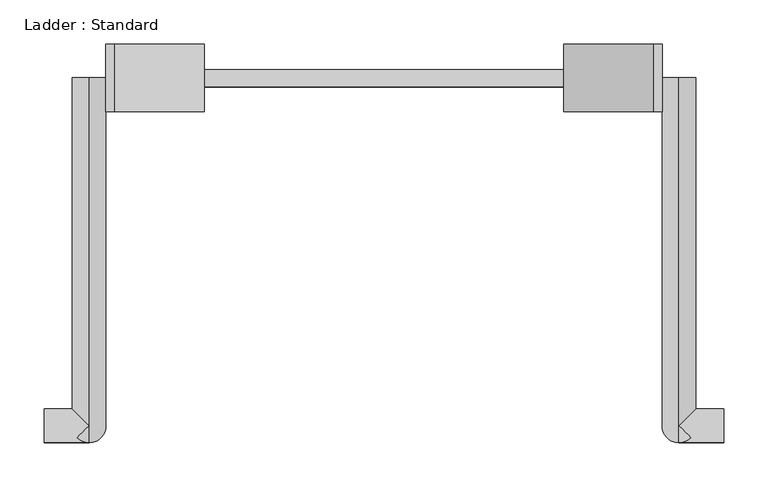
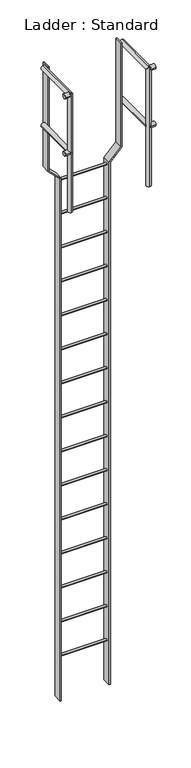
"""IFC4 building model written with IfcOpenShell, lengths in millimetres: proxy geometry, Ladder : Standard."""

import ifcopenshell
import ifcopenshell.guid

model = None  # the IFC model being written
_history = None  # IfcOwnerHistory: only IFC2X3 demands one
_inside = {}  # id of a spatial element -> (the spatial element, [elements in it])
_under = {}  # id of a project, library or spatial element -> (it, [spatial elements below it])
_declared = {}  # id of a project -> (the project, [libraries it declares])
_typed = {}  # id of a type object -> (the type object, [elements of that type])
_made_of = {}  # id of a material, layer set ... -> (it, [elements and type objects made of it])


def new_model(schema):
    """Start an empty IFC model of exactly this schema.

    Asked for "IFC4X3", IfcOpenShell would pick the latest addendum, in which some entities
    have other attributes; the version numbers below select the first issue.
    IFC2X3 requires an IfcOwnerHistory on every rooted entity: one is made here for all.
    """
    global model, _history
    if schema == "IFC4X3":
        model = ifcopenshell.file(schema_version=(4, 3, 0, 0))
    else:
        model = ifcopenshell.file(schema=schema)
    _inside.clear()
    _under.clear()
    _declared.clear()
    _typed.clear()
    _made_of.clear()
    _history = None
    if model.schema == "IFC2X3":
        org = make("IfcOrganization", Name="unknown")
        user = make(
            "IfcPersonAndOrganization",
            ThePerson=make("IfcPerson", FamilyName="unknown"),
            TheOrganization=org,
        )
        app = make(
            "IfcApplication",
            ApplicationDeveloper=org,
            Version="unknown",
            ApplicationFullName="unknown",
            ApplicationIdentifier="unknown",
        )
        _history = make(
            "IfcOwnerHistory",
            OwningUser=user,
            OwningApplication=app,
            ChangeAction="ADDED",
            CreationDate=0,
        )
    return model


def make(cls, **values):
    """One entity of the class cls with the attributes given. An attribute that is None is left unset."""
    return model.create_entity(
        cls, **{name: value for name, value in values.items() if value is not None}
    )


def rooted(cls, **values):
    """An entity with a GlobalId (a new one), such as an element, a storey or a relation."""
    return make(cls, GlobalId=ifcopenshell.guid.new(), OwnerHistory=_history, **values)


def si_unit(unit_type, name, prefix=None):
    """IfcSIUnit, for example si_unit("LENGTHUNIT", "METRE", prefix="MILLI")."""
    return make("IfcSIUnit", UnitType=unit_type, Prefix=prefix, Name=name)


def assignment(units):
    """IfcUnitAssignment: the units of a project."""
    return None if units is None else make("IfcUnitAssignment", Units=units)


def point(xyz):
    """IfcCartesianPoint."""
    return None if xyz is None else make("IfcCartesianPoint", Coordinates=xyz)


def direction(xyz):
    """IfcDirection."""
    return None if xyz is None else make("IfcDirection", DirectionRatios=xyz)


def frame(location, z_axis=None, x_axis=None):
    """IfcAxis2Placement3D, a coordinate frame: its origin and axes. An axis left out is left unset."""
    return make(
        "IfcAxis2Placement3D",
        Location=point(location),
        Axis=direction(z_axis),
        RefDirection=direction(x_axis),
    )


def frame_2d(location, x_axis=None):
    """IfcAxis2Placement2D, a coordinate frame in the plane: its origin and x axis."""
    return make(
        "IfcAxis2Placement2D", Location=point(location), RefDirection=direction(x_axis)
    )


def origin():
    """The frame at (0, 0, 0) with its axes left unset."""
    return frame((0.0, 0.0, 0.0))


def place(relative_to, where):
    """IfcLocalPlacement: puts the frame where relative to a parent placement (None: the world)."""
    return make(
        "IfcLocalPlacement", PlacementRelTo=relative_to, RelativePlacement=where
    )


def context(
    kind, dimensions, precision=None, world=None, true_north=None, identifier=None
):
    """IfcGeometricRepresentationContext, for example the 3D "Model" context."""
    return make(
        "IfcGeometricRepresentationContext",
        ContextIdentifier=identifier,
        ContextType=kind,
        CoordinateSpaceDimension=dimensions,
        Precision=precision,
        WorldCoordinateSystem=world,
        TrueNorth=true_north,
    )


def project(units=None, contexts=None):
    """IfcProject with its units and contexts."""
    return rooted(
        "IfcProject",
        Name="project",
        RepresentationContexts=contexts,
        UnitsInContext=assignment(units),
    )


def spatial(cls, under=None, at=None, **own):
    """A site, building, storey or space (cls), placed at a placement, below another one or the project."""
    s = rooted(cls, ObjectPlacement=at, **own)
    if under is not None:
        _under.setdefault(under.id(), (under, []))[1].append(s)
    return s


def polyline(points):
    """IfcPolyline through the points."""
    return make("IfcPolyline", Points=[point(p) for p in points])


def circle_curve(where, radius):
    """IfcCircle in the frame where."""
    return make("IfcCircle", Position=where, Radius=radius)


def ellipse_curve(where, semi_axis1, semi_axis2):
    """IfcEllipse in the frame where."""
    return make(
        "IfcEllipse", Position=where, SemiAxis1=semi_axis1, SemiAxis2=semi_axis2
    )


def trimmed(basis, trim1, trim2, sense, master):
    """IfcTrimmedCurve: the piece of a basis curve between two trims."""
    return make(
        "IfcTrimmedCurve",
        BasisCurve=basis,
        Trim1=trim1,
        Trim2=trim2,
        SenseAgreement=sense,
        MasterRepresentation=master,
    )


def segment(curve, same_sense, transition):
    """IfcCompositeCurveSegment."""
    return make(
        "IfcCompositeCurveSegment",
        Transition=transition,
        SameSense=same_sense,
        ParentCurve=curve,
    )


def composite_curve(segments, self_intersect=None):
    """IfcCompositeCurve: segments joined end to end."""
    return make("IfcCompositeCurve", Segments=segments, SelfIntersect=self_intersect)


def outline(outer, holes=None, kind="AREA"):
    """IfcArbitraryClosedProfileDef: a profile drawn as a closed curve; with holes, ...WithVoids."""
    if holes is None:
        return make("IfcArbitraryClosedProfileDef", ProfileType=kind, OuterCurve=outer)
    return make(
        "IfcArbitraryProfileDefWithVoids",
        ProfileType=kind,
        OuterCurve=outer,
        InnerCurves=holes,
    )


def extrude(swept, where, along, depth):
    """IfcExtrudedAreaSolid: the profile swept, set in the frame where, extruded along a direction by depth."""
    return make(
        "IfcExtrudedAreaSolid",
        SweptArea=swept,
        Position=where,
        ExtrudedDirection=direction(along),
        Depth=depth,
    )


def shape(context_of_items, identifier, shape_type, items):
    """IfcShapeRepresentation: the items that make up one representation, for example the "Body"."""
    return make(
        "IfcShapeRepresentation",
        ContextOfItems=context_of_items,
        RepresentationIdentifier=identifier,
        RepresentationType=shape_type,
        Items=items,
    )


def source(mapping_origin, context_of_items, identifier, shape_type, items):
    """IfcRepresentationMap: a shape defined once, which mapped items show again and again."""
    return make(
        "IfcRepresentationMap",
        MappingOrigin=mapping_origin,
        MappedRepresentation=shape(context_of_items, identifier, shape_type, items),
    )


def transform(
    local_origin,
    x_axis=None,
    y_axis=None,
    z_axis=None,
    scale=None,
    scale2=None,
    scale3=None,
    uniform=True,
):
    """IfcCartesianTransformationOperator3D, or its non-uniform kind. x_axis, y_axis, z_axis: its Axis1, 2, 3."""
    if uniform:
        return make(
            "IfcCartesianTransformationOperator3D",
            Axis1=direction(x_axis),
            Axis2=direction(y_axis),
            LocalOrigin=point(local_origin),
            Scale=scale,
            Axis3=direction(z_axis),
        )
    return make(
        "IfcCartesianTransformationOperator3DnonUniform",
        Axis1=direction(x_axis),
        Axis2=direction(y_axis),
        LocalOrigin=point(local_origin),
        Scale=scale,
        Axis3=direction(z_axis),
        Scale2=scale2,
        Scale3=scale3,
    )


def mapped(mapping_source, mapping_target):
    """IfcMappedItem: shows the shape of a source again, moved by a transform."""
    return make(
        "IfcMappedItem", MappingSource=mapping_source, MappingTarget=mapping_target
    )


def made_of(thing, what):
    """Note that an element or type object is made of a material, layer set ...; save() writes the relation."""
    if what is not None:
        _made_of.setdefault(what.id(), (what, []))[1].append(thing)
    return thing


def element(
    cls,
    number,
    at=None,
    inside=None,
    cuts=None,
    type_object=None,
    material=None,
    context=None,
    identifier="Body",
    shape_type=None,
    held_by="IfcProductDefinitionShape",
    body=None,
    shapes=None,
    **own,
):
    """One element of the class cls, such as IfcWall. Its Tag is "e" and its number.

    at: its placement. inside: the storey or other place that contains it. cuts: it is an
    opening in that element (IfcRelVoidsElement). A single representation is given by context,
    identifier, shape_type and body (its items); several are given by shapes. held_by: the class
    of the entity that holds the representations. save() writes the other relations.
    """
    e = rooted(cls, Tag="e%d" % number, ObjectPlacement=at, **own)
    if body is not None:
        shapes = [shape(context, identifier, shape_type, body)]
    if shapes is not None:
        e.Representation = make(held_by, Representations=shapes)
    if inside is not None:
        _inside.setdefault(inside.id(), (inside, []))[1].append(e)
    if cuts is not None:
        rooted(
            "IfcRelVoidsElement", RelatingBuildingElement=cuts, RelatedOpeningElement=e
        )
    if type_object is not None:
        _typed.setdefault(type_object.id(), (type_object, []))[1].append(e)
    return made_of(e, material)


def aggregate(whole, parts):
    """IfcRelAggregates: a whole, such as a stair, and the parts it consists of."""
    return rooted("IfcRelAggregates", RelatingObject=whole, RelatedObjects=parts)


def save(model, path):
    """Write the relations noted so far, then the file.

    IfcRelAggregates (storeys below a building ...), IfcRelContainedInSpatialStructure (elements
    in a storey), IfcRelDefinesByType, IfcRelAssociatesMaterial and IfcRelDeclares: one each for
    every whole, place, type object, material and project.
    """
    for whole, parts in _under.values():
        aggregate(whole, parts)
    for where, things in _inside.values():
        rooted(
            "IfcRelContainedInSpatialStructure",
            RelatedElements=things,
            RelatingStructure=where,
        )
    for kind, things in _typed.values():
        rooted("IfcRelDefinesByType", RelatedObjects=things, RelatingType=kind)
    for what, things in _made_of.values():
        rooted("IfcRelAssociatesMaterial", RelatedObjects=things, RelatingMaterial=what)
    for by, libraries in _declared.values():
        rooted("IfcRelDeclares", RelatingContext=by, RelatedDefinitions=libraries)
    model.write(path)


def plane_surface(at):
    """IfcPlane: the flat surface through the origin of the frame at, square to its z axis."""
    return make("IfcPlane", Position=at)


def cylinder_surface(at, radius):
    """IfcCylindricalSurface: all points at the distance radius from the z axis of the frame at."""
    return make("IfcCylindricalSurface", Position=at, Radius=radius)


def advanced_brep(points, edges, surfaces, faces):
    """IfcAdvancedBrep: a solid bounded by faces that lie on surfaces and meet in shared edges.

    An edge is (start, end): straight between two places in points (the first is 0);
    or (start, end, curve); or (start, end, curve, False) where it runs against its curve.
    A face is (place in surfaces, loops), or (place, loops, False) where it looks against
    its surface's normal. A loop lists edges by number (the first is 1), with a minus sign
    where the edge is run from its end to its start. The first loop is the outer one.
    """
    corners = [point(p) for p in points]
    vertices = [make("IfcVertexPoint", VertexGeometry=c) for c in corners]
    made = []
    for start, end, *more in edges:
        made.append(
            make(
                "IfcEdgeCurve",
                EdgeStart=vertices[start],
                EdgeEnd=vertices[end],
                EdgeGeometry=more[0] if more else make("IfcPolyline", Points=[corners[start], corners[end]]),
                SameSense=more[1] if len(more) > 1 else True,
            )
        )
    hull = []
    for where, loops, *sense in faces:
        bounds = []
        for j, loop in enumerate(loops):
            ring = [make("IfcOrientedEdge", EdgeElement=made[abs(k) - 1], Orientation=k > 0) for k in loop]
            bounds.append(
                make(
                    "IfcFaceOuterBound" if j == 0 else "IfcFaceBound",
                    Bound=make("IfcEdgeLoop", EdgeList=ring),
                    Orientation=True,
                )
            )
        hull.append(make("IfcAdvancedFace", Bounds=bounds, FaceSurface=surfaces[where], SameSense=sense[0] if sense else True))
    return make("IfcAdvancedBrep", Outer=make("IfcClosedShell", CfsFaces=hull))


def ladder_standard_9d180ee5(model_context):
    return source(origin(), model_context, "Body", "SolidModel", [
        extrude(outline(composite_curve([segment(trimmed(circle_curve(frame_2d((393.7, -4267.2)), 9.525), [point((384.175, -4267.2))], [point((403.225, -4267.2))], False, "CARTESIAN"), True, "CONTINUOUS"), segment(trimmed(circle_curve(frame_2d((393.7, -4267.2)), 9.525), [point((403.225, -4267.2))], [point((384.175, -4267.2))], False, "CARTESIAN"), True, "CONTINUOUS")], self_intersect=False)), frame((-203.2, 0.0, 0.0), z_axis=(1.0, 0.0, 0.0), x_axis=(0.0, 1.0, 0.0)), (0.0, 0.0, 1.0), 406.4),
        extrude(outline(composite_curve([segment(trimmed(circle_curve(frame_2d((393.7, -3962.4)), 9.525), [point((384.175, -3962.4))], [point((403.225, -3962.4))], False, "CARTESIAN"), True, "CONTINUOUS"), segment(trimmed(circle_curve(frame_2d((393.7, -3962.4)), 9.525), [point((403.225, -3962.4))], [point((384.175, -3962.4))], False, "CARTESIAN"), True, "CONTINUOUS")], self_intersect=False)), frame((-203.2, 0.0, 0.0), z_axis=(1.0, 0.0, 0.0), x_axis=(0.0, 1.0, 0.0)), (0.0, 0.0, 1.0), 406.4),
        extrude(outline(composite_curve([segment(trimmed(circle_curve(frame_2d((393.7, -3657.6)), 9.525), [point((384.175, -3657.6))], [point((403.225, -3657.6))], False, "CARTESIAN"), True, "CONTINUOUS"), segment(trimmed(circle_curve(frame_2d((393.7, -3657.6)), 9.525), [point((403.225, -3657.6))], [point((384.175, -3657.6))], False, "CARTESIAN"), True, "CONTINUOUS")], self_intersect=False)), frame((-203.2, 0.0, 0.0), z_axis=(1.0, 0.0, 0.0), x_axis=(0.0, 1.0, 0.0)), (0.0, 0.0, 1.0), 406.4),
        extrude(outline(composite_curve([segment(trimmed(circle_curve(frame_2d((393.7, -3352.8)), 9.525), [point((384.175, -3352.8))], [point((403.225, -3352.8))], False, "CARTESIAN"), True, "CONTINUOUS"), segment(trimmed(circle_curve(frame_2d((393.7, -3352.8)), 9.525), [point((403.225, -3352.8))], [point((384.175, -3352.8))], False, "CARTESIAN"), True, "CONTINUOUS")], self_intersect=False)), frame((-203.2, 0.0, 0.0), z_axis=(1.0, 0.0, 0.0), x_axis=(0.0, 1.0, 0.0)), (0.0, 0.0, 1.0), 406.4),
        extrude(outline(composite_curve([segment(trimmed(circle_curve(frame_2d((393.7, -3048.0)), 9.525), [point((384.175, -3048.0))], [point((403.225, -3048.0))], False, "CARTESIAN"), True, "CONTINUOUS"), segment(trimmed(circle_curve(frame_2d((393.7, -3048.0)), 9.525), [point((403.225, -3048.0))], [point((384.175, -3048.0))], False, "CARTESIAN"), True, "CONTINUOUS")], self_intersect=False)), frame((-203.2, 0.0, 0.0), z_axis=(1.0, 0.0, 0.0), x_axis=(0.0, 1.0, 0.0)), (0.0, 0.0, 1.0), 406.4),
        extrude(outline(composite_curve([segment(trimmed(circle_curve(frame_2d((393.7, -2743.2)), 9.525), [point((384.175, -2743.2))], [point((403.225, -2743.2))], False, "CARTESIAN"), True, "CONTINUOUS"), segment(trimmed(circle_curve(frame_2d((393.7, -2743.2)), 9.525), [point((403.225, -2743.2))], [point((384.175, -2743.2))], False, "CARTESIAN"), True, "CONTINUOUS")], self_intersect=False)), frame((-203.2, 0.0, 0.0), z_axis=(1.0, 0.0, 0.0), x_axis=(0.0, 1.0, 0.0)), (0.0, 0.0, 1.0), 406.4),
        extrude(outline(composite_curve([segment(trimmed(circle_curve(frame_2d((393.7, -2438.4)), 9.525), [point((384.175, -2438.4))], [point((403.225, -2438.4))], False, "CARTESIAN"), True, "CONTINUOUS"), segment(trimmed(circle_curve(frame_2d((393.7, -2438.4)), 9.525), [point((403.225, -2438.4))], [point((384.175, -2438.4))], False, "CARTESIAN"), True, "CONTINUOUS")], self_intersect=False)), frame((-203.2, 0.0, 0.0), z_axis=(1.0, 0.0, 0.0), x_axis=(0.0, 1.0, 0.0)), (0.0, 0.0, 1.0), 406.4),
        extrude(outline(composite_curve([segment(trimmed(circle_curve(frame_2d((393.7, -2133.6)), 9.525), [point((384.175, -2133.6))], [point((403.225, -2133.6))], False, "CARTESIAN"), True, "CONTINUOUS"), segment(trimmed(circle_curve(frame_2d((393.7, -2133.6)), 9.525), [point((403.225, -2133.6))], [point((384.175, -2133.6))], False, "CARTESIAN"), True, "CONTINUOUS")], self_intersect=False)), frame((-203.2, 0.0, 0.0), z_axis=(1.0, 0.0, 0.0), x_axis=(0.0, 1.0, 0.0)), (0.0, 0.0, 1.0), 406.4),
        extrude(outline(composite_curve([segment(trimmed(circle_curve(frame_2d((393.7, -1828.8)), 9.525), [point((384.175, -1828.8))], [point((403.225, -1828.8))], False, "CARTESIAN"), True, "CONTINUOUS"), segment(trimmed(circle_curve(frame_2d((393.7, -1828.8)), 9.525), [point((403.225, -1828.8))], [point((384.175, -1828.8))], False, "CARTESIAN"), True, "CONTINUOUS")], self_intersect=False)), frame((-203.2, 0.0, 0.0), z_axis=(1.0, 0.0, 0.0), x_axis=(0.0, 1.0, 0.0)), (0.0, 0.0, 1.0), 406.4),
        extrude(outline(composite_curve([segment(trimmed(circle_curve(frame_2d((393.7, -1524.0)), 9.525), [point((384.175, -1524.0))], [point((403.225, -1524.0))], False, "CARTESIAN"), True, "CONTINUOUS"), segment(trimmed(circle_curve(frame_2d((393.7, -1524.0)), 9.525), [point((403.225, -1524.0))], [point((384.175, -1524.0))], False, "CARTESIAN"), True, "CONTINUOUS")], self_intersect=False)), frame((-203.2, 0.0, 0.0), z_axis=(1.0, 0.0, 0.0), x_axis=(0.0, 1.0, 0.0)), (0.0, 0.0, 1.0), 406.4),
        extrude(outline(composite_curve([segment(trimmed(circle_curve(frame_2d((393.7, -1219.2)), 9.525), [point((384.175, -1219.2))], [point((403.225, -1219.2))], False, "CARTESIAN"), True, "CONTINUOUS"), segment(trimmed(circle_curve(frame_2d((393.7, -1219.2)), 9.525), [point((403.225, -1219.2))], [point((384.175, -1219.2))], False, "CARTESIAN"), True, "CONTINUOUS")], self_intersect=False)), frame((-203.2, 0.0, 0.0), z_axis=(1.0, 0.0, 0.0), x_axis=(0.0, 1.0, 0.0)), (0.0, 0.0, 1.0), 406.4),
        extrude(outline(composite_curve([segment(trimmed(circle_curve(frame_2d((393.7, -914.4)), 9.525), [point((384.175, -914.4))], [point((403.225, -914.4))], False, "CARTESIAN"), True, "CONTINUOUS"), segment(trimmed(circle_curve(frame_2d((393.7, -914.4)), 9.525), [point((403.225, -914.4))], [point((384.175, -914.4))], False, "CARTESIAN"), True, "CONTINUOUS")], self_intersect=False)), frame((-203.2, 0.0, 0.0), z_axis=(1.0, 0.0, 0.0), x_axis=(0.0, 1.0, 0.0)), (0.0, 0.0, 1.0), 406.4),
        extrude(outline(composite_curve([segment(trimmed(circle_curve(frame_2d((393.7, -609.6)), 9.525), [point((384.175, -609.6))], [point((403.225, -609.6))], False, "CARTESIAN"), True, "CONTINUOUS"), segment(trimmed(circle_curve(frame_2d((393.7, -609.6)), 9.525), [point((403.225, -609.6))], [point((384.175, -609.6))], False, "CARTESIAN"), True, "CONTINUOUS")], self_intersect=False)), frame((-203.2, 0.0, 0.0), z_axis=(1.0, 0.0, 0.0), x_axis=(0.0, 1.0, 0.0)), (0.0, 0.0, 1.0), 406.4),
        extrude(outline(composite_curve([segment(trimmed(circle_curve(frame_2d((393.7, -304.8)), 9.525), [point((384.175, -304.8))], [point((403.225, -304.8))], False, "CARTESIAN"), True, "CONTINUOUS"), segment(trimmed(circle_curve(frame_2d((393.7, -304.8)), 9.525), [point((403.225, -304.8))], [point((384.175, -304.8))], False, "CARTESIAN"), True, "CONTINUOUS")], self_intersect=False)), frame((-203.2, 0.0, 0.0), z_axis=(1.0, 0.0, 0.0), x_axis=(0.0, 1.0, 0.0)), (0.0, 0.0, 1.0), 406.4),
        extrude(outline(composite_curve([segment(trimmed(circle_curve(frame_2d((393.7, 0.0)), 9.525), [point((384.175, 0.0))], [point((403.225, 0.0))], False, "CARTESIAN"), True, "CONTINUOUS"), segment(trimmed(circle_curve(frame_2d((393.7, 0.0)), 9.525), [point((403.225, 0.0))], [point((384.175, 0.0))], False, "CARTESIAN"), True, "CONTINUOUS")], self_intersect=False)), frame((-203.2, 0.0, 0.0), z_axis=(1.0, 0.0, 0.0), x_axis=(0.0, 1.0, 0.0)), (0.0, 0.0, 1.0), 406.4),
        advanced_brep(
        [(314.325, 393.7, 533.4), (352.425, 393.7, 533.4), (352.425, 19.05, 533.4), (346.8453842, 13.4703842, 519.9296158), (333.375, 19.05, 514.35), (314.325, 0.0, 533.4), (333.375, 19.05, 552.45), (346.8453842, 13.4703842, 546.8703842), (384.175, -19.05, 533.4), (384.175, 19.05, 533.4), (333.375, -19.05, 533.4), (333.375, 19.05, 0.0), (333.375, -19.05, 0.0), (333.375, 19.05, 1028.7), (346.8453842, 13.4703842, 1034.2796158), (333.375, -19.05, 1047.75), (346.8453842, -13.4703842, 1061.2203842), (333.375, -19.05, 1066.8), (333.375, 393.7, 1028.7), (333.375, 393.7, 1066.8), (333.375, 0.0, 1066.8), (352.425, 19.05, 1047.75), (384.175, -19.05, 1047.75), (384.175, 19.05, 1047.75)],
        [
            (0, 1, circle_curve(frame((333.375, 393.7, 533.4), z_axis=(0.0, 1.0, 0.0), x_axis=(1.0, 0.0, 0.0)), 19.05)),
            (1, 0, circle_curve(frame((333.375, 393.7, 533.4), z_axis=(0.0, 1.0, 0.0), x_axis=(1.0, 0.0, 0.0)), 19.05)),
            (1, 2),
            (2, 3, ellipse_curve(frame((333.375, 0.0, 533.4), z_axis=(-0.7071067811865459, 0.7071067811865492, 0.0), x_axis=(-0.7071067811865492, -0.7071067811865457, 0.0)), 26.9407684, 19.05)),
            (3, 4, ellipse_curve(frame((333.375, 0.0, 533.4), z_axis=(0.0, 0.7071067811865475, 0.7071067811865475), x_axis=(0.0, -0.7071067811865476, 0.7071067811865474)), 26.9407684, 19.05)),
            (4, 5, ellipse_curve(frame((333.375, 0.0, 533.4), z_axis=(0.0, 0.7071067811865475, 0.7071067811865475), x_axis=(0.0, -0.7071067811865476, 0.7071067811865474)), 26.9407684, 19.05)),
            (5, 0),
            (5, 6, ellipse_curve(frame((333.375, 0.0, 533.4), z_axis=(0.0, 0.7071067811865475, -0.7071067811865475), x_axis=(0.0, -0.7071067811865476, -0.7071067811865474)), 26.9407684, 19.05)),
            (6, 7, ellipse_curve(frame((333.375, 0.0, 533.4), z_axis=(0.0, 0.7071067811865475, -0.7071067811865475), x_axis=(0.0, -0.7071067811865476, -0.7071067811865474)), 26.9407684, 19.05)),
            (7, 2, ellipse_curve(frame((333.375, 0.0, 533.4), z_axis=(-0.7071067811865459, 0.7071067811865492, 0.0), x_axis=(-0.7071067811865492, -0.7071067811865457, 0.0)), 26.9407684, 19.05)),
            (8, 9, circle_curve(frame((384.175, 0.0, 533.4), z_axis=(1.0, 0.0, 0.0), x_axis=(0.0, 1.0, 0.0)), 19.05)),
            (9, 8, circle_curve(frame((384.175, 0.0, 533.4), z_axis=(1.0, 0.0, 0.0), x_axis=(0.0, 1.0, 0.0)), 19.05)),
            (8, 10),
            (10, 3, ellipse_curve(frame((333.375, 0.0, 533.4), z_axis=(0.7071067811865475, 0.0, 0.7071067811865476), x_axis=(0.7071067811865476, 0.0, -0.7071067811865474)), 26.9407684, 19.05)),
            (2, 9),
            (7, 10, ellipse_curve(frame((333.375, 0.0, 533.4), z_axis=(0.7071067811865476, 0.0, -0.7071067811865475), x_axis=(0.7071067811865474, 0.0, 0.7071067811865476)), 26.9407684, 19.05)),
            (11, 12, circle_curve(frame((333.375, 0.0, 0.0), z_axis=(0.0, 0.0, -1.0), x_axis=(0.0, -1.0, 0.0)), 19.05)),
            (12, 11, circle_curve(frame((333.375, 0.0, 0.0), z_axis=(0.0, 0.0, -1.0), x_axis=(0.0, -1.0, 0.0)), 19.05)),
            (11, 4),
            (10, 12),
            (6, 13),
            (13, 14, ellipse_curve(frame((333.375, 0.0, 1047.75), z_axis=(0.0, -0.7071067811865475, -0.7071067811865475), x_axis=(0.0, 0.7071067811865474, -0.7071067811865476)), 26.9407684, 19.05)),
            (14, 15, ellipse_curve(frame((333.375, 0.0, 1047.75), z_axis=(-0.7071067811865475, 0.0, -0.7071067811865476), x_axis=(0.7071067811865476, 0.0, -0.7071067811865474)), 26.9407684, 19.05)),
            (15, 10),
            (16, 17, ellipse_curve(frame((333.375, 0.0, 1047.75), z_axis=(0.0, -0.7071067811865475, -0.7071067811865475), x_axis=(0.0, 0.7071067811865474, -0.7071067811865476)), 26.9407684, 19.05)),
            (17, 15),
            (15, 16, ellipse_curve(frame((333.375, 0.0, 1047.75), z_axis=(-0.7071067811865476, 0.0, 0.7071067811865475), x_axis=(-0.7071067811865474, 0.0, -0.7071067811865476)), 26.9407684, 19.05)),
            (17, 13, ellipse_curve(frame((333.375, 0.0, 1047.75), z_axis=(0.0, -0.7071067811865475, -0.7071067811865475), x_axis=(0.0, 0.7071067811865474, -0.7071067811865476)), 26.9407684, 19.05)),
            (18, 19, circle_curve(frame((333.375, 393.7, 1047.75), z_axis=(0.0, 1.0, 0.0), x_axis=(0.0, 0.0, 1.0)), 19.05)),
            (19, 18, circle_curve(frame((333.375, 393.7, 1047.75), z_axis=(0.0, 1.0, 0.0), x_axis=(0.0, 0.0, 1.0)), 19.05)),
            (16, 20, ellipse_curve(frame((333.375, 0.0, 1047.75), z_axis=(-0.7071067811865508, -0.7071067811865441, 0.0), x_axis=(0.7071067811865441, -0.7071067811865509, 0.0)), 26.9407684, 19.05)),
            (20, 17),
            (19, 20),
            (20, 21, ellipse_curve(frame((333.375, 0.0, 1047.75), z_axis=(-0.7071067811865441, 0.7071067811865508, 0.0), x_axis=(-0.7071067811865507, -0.7071067811865442, 0.0)), 26.9407684, 19.05)),
            (21, 14, ellipse_curve(frame((333.375, 0.0, 1047.75), z_axis=(-0.7071067811865441, 0.7071067811865508, 0.0), x_axis=(-0.7071067811865507, -0.7071067811865442, 0.0)), 26.9407684, 19.05)),
            (13, 18),
            (22, 23, circle_curve(frame((384.175, 0.0, 1047.75), z_axis=(1.0, 0.0, 0.0), x_axis=(0.0, 1.0, 0.0)), 19.05)),
            (23, 22, circle_curve(frame((384.175, 0.0, 1047.75), z_axis=(1.0, 0.0, 0.0), x_axis=(0.0, 1.0, 0.0)), 19.05)),
            (22, 15),
            (21, 23),
        ],
        [
            plane_surface(frame((352.425, 393.7, 533.4), z_axis=(0.0, 1.0, 0.0), x_axis=(0.0, 0.0, -1.0))),
            cylinder_surface(frame((333.375, 393.7, 533.4), z_axis=(0.0, -1.0, 0.0), x_axis=(1.0, 0.0, 0.0)), 19.05),
            plane_surface(frame((384.175, 19.05, 533.4), z_axis=(1.0, 0.0, 0.0), x_axis=(0.0, 0.0, 1.0))),
            cylinder_surface(frame((333.375, 0.0, 533.4), z_axis=(1.0, 0.0, 0.0), x_axis=(0.0, 1.0, 0.0)), 19.05),
            plane_surface(frame((0.0, 0.0, 0.0), z_axis=(0.0, 0.0, -1.0), x_axis=(1.0, 0.0, 0.0))),
            cylinder_surface(frame((333.375, 0.0, 0.0), z_axis=(0.0, 0.0, -1.0), x_axis=(0.0, -1.0, 0.0)), 19.05),
            plane_surface(frame((0.0, 393.7, 1047.75), z_axis=(0.0, 1.0, 0.0), x_axis=(1.0, 0.0, 0.0))),
            cylinder_surface(frame((333.375, 0.0, 1047.75), z_axis=(0.0, -1.0, 0.0), x_axis=(0.0, 0.0, 1.0)), 19.05),
            plane_surface(frame((384.175, 19.05, 1047.75), z_axis=(1.0, 0.0, 0.0), x_axis=(0.0, 0.0, 1.0))),
            cylinder_surface(frame((333.375, 0.0, 1047.75), z_axis=(1.0, 0.0, 0.0), x_axis=(0.0, 1.0, 0.0)), 19.05),
        ],
        [
            (0, [[1, 2]]),
            (1, [[-2, 3, 4, 5, 6, 7]]),
            (1, [[-1, -7, 8, 9, 10, -3]]),
            (2, [[11, 12]]),
            (3, [[-11, 13, 14, -4, 15]]),
            (3, [[-12, -15, -10, 16, -13]]),
            (4, [[17, 18]]),
            (5, [[-17, 19, -5, -14, 20]]),
            (5, [[21, 22, 23, 24, -16, -9]]),
            (5, [[25, 26, 27]]),
            (5, [[-18, -20, -24, -26, 28, -21, -8, -6, -19]]),
            (6, [[29, 30]]),
            (7, [[-25, 31, 32]]),
            (7, [[-30, 33, 34, 35, -22, 36]]),
            (7, [[-28, -32, -33, -29, -36]]),
            (8, [[37, 38]]),
            (9, [[-37, 39, -23, -35, 40]]),
            (9, [[-38, -40, -34, -31, -27, -39]]),
        ],
    ),
        advanced_brep(
        [(-384.175, -19.05, 533.4), (-384.175, 19.05, 533.4), (-352.425, 19.05, 533.4), (-346.8453842, 13.4703842, 519.9296158), (-333.375, -19.05, 533.4), (-346.8453842, 13.4703842, 546.8703842), (-352.425, 393.7, 533.4), (-314.325, 393.7, 533.4), (-314.325, 0.0, 533.4), (-333.375, 19.05, 514.35), (-333.375, 19.05, 552.45), (-333.375, 19.05, 0.0), (-333.375, -19.05, 0.0), (-333.375, 19.05, 1028.7), (-333.375, -19.05, 1066.8), (-333.375, -19.05, 1047.75), (-346.8453842, 13.4703842, 1034.2796158), (-346.8453842, -13.4703842, 1061.2203842), (-333.375, 393.7, 1028.7), (-333.375, 393.7, 1066.8), (-333.375, 0.0, 1066.8), (-352.425, 19.05, 1047.75), (-384.175, -19.05, 1047.75), (-384.175, 19.05, 1047.75)],
        [
            (0, 1, circle_curve(frame((-384.175, 0.0, 533.4), z_axis=(-1.0, 0.0, 0.0), x_axis=(0.0, 1.0, 0.0)), 19.05)),
            (1, 0, circle_curve(frame((-384.175, 0.0, 533.4), z_axis=(-1.0, 0.0, 0.0), x_axis=(0.0, 1.0, 0.0)), 19.05)),
            (1, 2),
            (2, 3, ellipse_curve(frame((-333.375, 0.0, 533.4), z_axis=(-0.7071067811865491, -0.7071067811865458, 0.0), x_axis=(0.7071067811865459, -0.707106781186549, 0.0)), 26.9407684, 19.05)),
            (3, 4, ellipse_curve(frame((-333.375, 0.0, 533.4), z_axis=(-0.7071067811865476, 0.0, 0.7071067811865475), x_axis=(0.7071067811865474, 0.0, 0.7071067811865476)), 26.9407684, 19.05)),
            (4, 0),
            (4, 5, ellipse_curve(frame((-333.375, 0.0, 533.4), z_axis=(-0.7071067811865475, 0.0, -0.7071067811865476), x_axis=(0.7071067811865476, 0.0, -0.7071067811865474)), 26.9407684, 19.05)),
            (5, 2, ellipse_curve(frame((-333.375, 0.0, 533.4), z_axis=(-0.7071067811865491, -0.7071067811865458, 0.0), x_axis=(0.7071067811865459, -0.707106781186549, 0.0)), 26.9407684, 19.05)),
            (6, 7, circle_curve(frame((-333.375, 393.7, 533.4), z_axis=(0.0, 1.0, 0.0), x_axis=(1.0, 0.0, 0.0)), 19.05)),
            (7, 6, circle_curve(frame((-333.375, 393.7, 533.4), z_axis=(0.0, 1.0, 0.0), x_axis=(1.0, 0.0, 0.0)), 19.05)),
            (7, 8),
            (8, 9, ellipse_curve(frame((-333.375, 0.0, 533.4), z_axis=(0.0, 0.7071067811865475, 0.7071067811865475), x_axis=(0.0, -0.7071067811865476, 0.7071067811865474)), 26.9407684, 19.05)),
            (9, 3, ellipse_curve(frame((-333.375, 0.0, 533.4), z_axis=(0.0, 0.7071067811865475, 0.7071067811865475), x_axis=(0.0, -0.7071067811865476, 0.7071067811865474)), 26.9407684, 19.05)),
            (2, 6),
            (5, 10, ellipse_curve(frame((-333.375, 0.0, 533.4), z_axis=(0.0, 0.7071067811865475, -0.7071067811865475), x_axis=(0.0, -0.7071067811865476, -0.7071067811865474)), 26.9407684, 19.05)),
            (10, 8, ellipse_curve(frame((-333.375, 0.0, 533.4), z_axis=(0.0, 0.7071067811865475, -0.7071067811865475), x_axis=(0.0, -0.7071067811865476, -0.7071067811865474)), 26.9407684, 19.05)),
            (11, 12, circle_curve(frame((-333.375, 0.0, 0.0), z_axis=(0.0, 0.0, -1.0), x_axis=(0.0, -1.0, 0.0)), 19.05)),
            (12, 11, circle_curve(frame((-333.375, 0.0, 0.0), z_axis=(0.0, 0.0, -1.0), x_axis=(0.0, -1.0, 0.0)), 19.05)),
            (11, 9),
            (10, 13),
            (13, 14, ellipse_curve(frame((-333.375, 0.0, 1047.75), z_axis=(0.0, -0.7071067811865475, -0.7071067811865475), x_axis=(0.0, 0.7071067811865474, -0.7071067811865476)), 26.9407684, 19.05)),
            (14, 15),
            (15, 4),
            (4, 12),
            (15, 16, ellipse_curve(frame((-333.375, 0.0, 1047.75), z_axis=(0.7071067811865476, 0.0, -0.7071067811865475), x_axis=(-0.7071067811865474, 0.0, -0.7071067811865476)), 26.9407684, 19.05)),
            (16, 13, ellipse_curve(frame((-333.375, 0.0, 1047.75), z_axis=(0.0, -0.7071067811865475, -0.7071067811865475), x_axis=(0.0, 0.7071067811865474, -0.7071067811865476)), 26.9407684, 19.05)),
            (14, 17, ellipse_curve(frame((-333.375, 0.0, 1047.75), z_axis=(0.0, -0.7071067811865475, -0.7071067811865475), x_axis=(0.0, 0.7071067811865474, -0.7071067811865476)), 26.9407684, 19.05)),
            (17, 15, ellipse_curve(frame((-333.375, 0.0, 1047.75), z_axis=(0.7071067811865475, 0.0, 0.7071067811865476), x_axis=(0.7071067811865476, 0.0, -0.7071067811865474)), 26.9407684, 19.05)),
            (18, 19, circle_curve(frame((-333.375, 393.7, 1047.75), z_axis=(0.0, 1.0, 0.0), x_axis=(0.0, 0.0, 1.0)), 19.05)),
            (19, 18, circle_curve(frame((-333.375, 393.7, 1047.75), z_axis=(0.0, 1.0, 0.0), x_axis=(0.0, 0.0, 1.0)), 19.05)),
            (13, 18),
            (19, 20),
            (20, 14),
            (20, 17, ellipse_curve(frame((-333.375, 0.0, 1047.75), z_axis=(0.7071067811865441, -0.7071067811865508, 0.0), x_axis=(-0.7071067811865507, -0.7071067811865442, 0.0)), 26.9407684, 19.05)),
            (16, 21, ellipse_curve(frame((-333.375, 0.0, 1047.75), z_axis=(0.7071067811865508, 0.7071067811865441, 0.0), x_axis=(0.7071067811865441, -0.7071067811865509, 0.0)), 26.9407684, 19.05)),
            (21, 20, ellipse_curve(frame((-333.375, 0.0, 1047.75), z_axis=(0.7071067811865508, 0.7071067811865441, 0.0), x_axis=(0.7071067811865441, -0.7071067811865509, 0.0)), 26.9407684, 19.05)),
            (22, 23, circle_curve(frame((-384.175, 0.0, 1047.75), z_axis=(-1.0, 0.0, 0.0), x_axis=(0.0, 1.0, 0.0)), 19.05)),
            (23, 22, circle_curve(frame((-384.175, 0.0, 1047.75), z_axis=(-1.0, 0.0, 0.0), x_axis=(0.0, 1.0, 0.0)), 19.05)),
            (23, 21),
            (15, 22),
        ],
        [
            plane_surface(frame((-384.175, 19.05, 533.4), z_axis=(-1.0, 0.0, 0.0), x_axis=(0.0, 0.0, -1.0))),
            cylinder_surface(frame((-384.175, 0.0, 533.4), z_axis=(1.0, 0.0, 0.0), x_axis=(0.0, 1.0, 0.0)), 19.05),
            plane_surface(frame((-314.325, 393.7, 533.4), z_axis=(0.0, 1.0, 0.0), x_axis=(0.0, 0.0, -1.0))),
            cylinder_surface(frame((-333.375, 393.7, 533.4), z_axis=(0.0, -1.0, 0.0), x_axis=(1.0, 0.0, 0.0)), 19.05),
            plane_surface(frame((0.0, 0.0, 0.0), z_axis=(0.0, 0.0, -1.0), x_axis=(1.0, 0.0, 0.0))),
            cylinder_surface(frame((-333.375, 0.0, 0.0), z_axis=(0.0, 0.0, -1.0), x_axis=(0.0, -1.0, 0.0)), 19.05),
            plane_surface(frame((0.0, 393.7, 1047.75), z_axis=(0.0, 1.0, 0.0), x_axis=(1.0, 0.0, 0.0))),
            cylinder_surface(frame((-333.375, 0.0, 1047.75), z_axis=(0.0, -1.0, 0.0), x_axis=(0.0, 0.0, 1.0)), 19.05),
            plane_surface(frame((-384.175, 19.05, 1047.75), z_axis=(-1.0, 0.0, 0.0), x_axis=(0.0, 0.0, -1.0))),
            cylinder_surface(frame((-384.175, 0.0, 1047.75), z_axis=(1.0, 0.0, 0.0), x_axis=(0.0, 1.0, 0.0)), 19.05),
        ],
        [
            (0, [[1, 2]]),
            (1, [[-2, 3, 4, 5, 6]]),
            (1, [[-1, -6, 7, 8, -3]]),
            (2, [[9, 10]]),
            (3, [[-10, 11, 12, 13, -4, 14]]),
            (3, [[-9, -14, -8, 15, 16, -11]]),
            (4, [[17, 18]]),
            (5, [[-17, 19, -12, -16, 20, 21, 22, 23, 24]]),
            (5, [[-18, -24, -5, -13, -19]]),
            (5, [[-20, -15, -7, -23, 25, 26]]),
            (5, [[27, 28, -22]]),
            (6, [[29, 30]]),
            (7, [[-21, 31, -30, 32, 33]]),
            (7, [[-27, -33, 34]]),
            (7, [[-29, -31, -26, 35, 36, -32]]),
            (8, [[37, 38]]),
            (9, [[-38, 39, -35, -25, 40]]),
            (9, [[-37, -40, -28, -34, -36, -39]]),
        ],
    ),
        extrude(outline(polyline([(1066.8, -314.325), (133.35, -314.325), (31.75, -212.725), (-4648.2, -212.725), (-4648.2, -203.2), (35.6953842, -203.2), (137.2953842, -304.8), (1066.8, -304.8), (1066.8, -314.325)])), frame((0.0, 355.6, 0.0), z_axis=(0.0, 1.0, 0.0), x_axis=(0.0, 0.0, 1.0)), (0.0, 0.0, 1.0), 76.2),
        extrude(outline(polyline([(1066.8, 304.8), (137.2953842, 304.8), (35.6953842, 203.2), (-4648.2, 203.2), (-4648.2, 212.725), (31.75, 212.725), (133.35, 314.325), (1066.8, 314.325), (1066.8, 304.8)])), frame((0.0, 355.6, 0.0), z_axis=(0.0, 1.0, 0.0), x_axis=(0.0, 0.0, 1.0)), (0.0, 0.0, 1.0), 76.2),
    ])


if __name__ == "__main__":
    model = new_model("IFC4")
    model_context = context("Model", 3, world=origin())
    ifc_project = project(units=[si_unit("LENGTHUNIT", "METRE", prefix="MILLI")], contexts=[model_context])
    site = spatial("IfcSite", under=ifc_project)
    building = spatial("IfcBuilding", under=site)
    placement = place(None, origin())
    ladder_standard_shape = ladder_standard_9d180ee5(model_context)
    element("IfcBuildingElementProxy", 1, Name="Ladder : Standard", ObjectType="Ladder : Standard", at=placement, inside=building, context=model_context, shape_type="MappedRepresentation", body=[
        mapped(ladder_standard_shape, transform((0.0, 0.0, 0.0), x_axis=(1.0, 0.0, 0.0), y_axis=(0.0, 1.0, 0.0), z_axis=(0.0, 0.0, 1.0))),
    ])
    save(model, "model.ifc")

# Revit data of these elements
# Type "Ladder : Standard"
#   Rung Radius = 0' - 0 3/8"
#   Rung Length [instance default] = 1' - 4"
#   Side Rail Thickness = 0' - 3"
#   Side Rail Width = 0' - 0 3/8"
#   Half Guardrail Height = 1' - 9"
#   Height [instance default] = 15' - 2 1/2"
#   Guardrail Length = 0' - 2"
#   Guardrail Height = 3' - 6"
#   Distance [instance default] = 0' - 7"
#   Rung Space [instance default] = 1' - 0"
#   Number of Rungs [instance default] = 15
#   Default Elevation = 0
# Element 1 (IfcBuildingElementProxy, "Ladder : Standard")
#   Height = 15' - 3"
